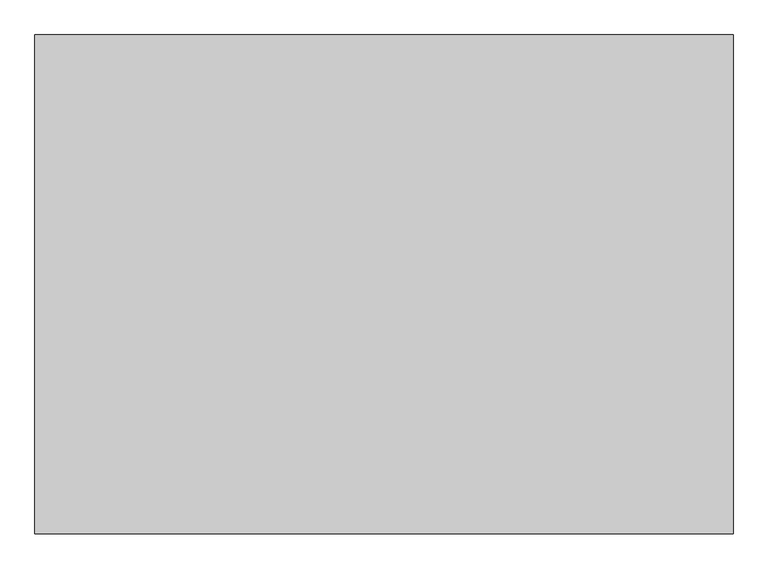
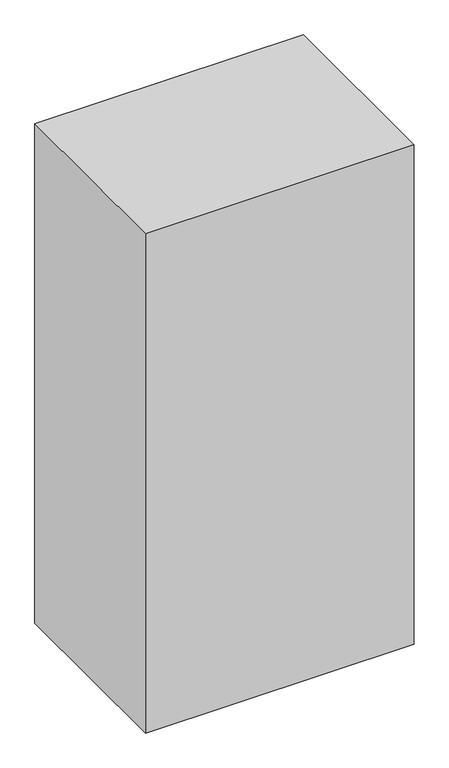
"""IFC4 building model written with IfcOpenShell, lengths in millimetres: proxy geometry, Space Planning Box_hec : Space Planning Box_hec."""

import ifcopenshell
import ifcopenshell.guid

model = None  # the IFC model being written
_history = None  # IfcOwnerHistory: only IFC2X3 demands one
_inside = {}  # id of a spatial element -> (the spatial element, [elements in it])
_under = {}  # id of a project, library or spatial element -> (it, [spatial elements below it])
_declared = {}  # id of a project -> (the project, [libraries it declares])
_typed = {}  # id of a type object -> (the type object, [elements of that type])
_made_of = {}  # id of a material, layer set ... -> (it, [elements and type objects made of it])


def new_model(schema):
    """Start an empty IFC model of exactly this schema.

    Asked for "IFC4X3", IfcOpenShell would pick the latest addendum, in which some entities
    have other attributes; the version numbers below select the first issue.
    IFC2X3 requires an IfcOwnerHistory on every rooted entity: one is made here for all.
    """
    global model, _history
    if schema == "IFC4X3":
        model = ifcopenshell.file(schema_version=(4, 3, 0, 0))
    else:
        model = ifcopenshell.file(schema=schema)
    _inside.clear()
    _under.clear()
    _declared.clear()
    _typed.clear()
    _made_of.clear()
    _history = None
    if model.schema == "IFC2X3":
        org = make("IfcOrganization", Name="unknown")
        user = make(
            "IfcPersonAndOrganization",
            ThePerson=make("IfcPerson", FamilyName="unknown"),
            TheOrganization=org,
        )
        app = make(
            "IfcApplication",
            ApplicationDeveloper=org,
            Version="unknown",
            ApplicationFullName="unknown",
            ApplicationIdentifier="unknown",
        )
        _history = make(
            "IfcOwnerHistory",
            OwningUser=user,
            OwningApplication=app,
            ChangeAction="ADDED",
            CreationDate=0,
        )
    return model


def make(cls, **values):
    """One entity of the class cls with the attributes given. An attribute that is None is left unset."""
    return model.create_entity(
        cls, **{name: value for name, value in values.items() if value is not None}
    )


def rooted(cls, **values):
    """An entity with a GlobalId (a new one), such as an element, a storey or a relation."""
    return make(cls, GlobalId=ifcopenshell.guid.new(), OwnerHistory=_history, **values)


def si_unit(unit_type, name, prefix=None):
    """IfcSIUnit, for example si_unit("LENGTHUNIT", "METRE", prefix="MILLI")."""
    return make("IfcSIUnit", UnitType=unit_type, Prefix=prefix, Name=name)


def assignment(units):
    """IfcUnitAssignment: the units of a project."""
    return None if units is None else make("IfcUnitAssignment", Units=units)


def point(xyz):
    """IfcCartesianPoint."""
    return None if xyz is None else make("IfcCartesianPoint", Coordinates=xyz)


def direction(xyz):
    """IfcDirection."""
    return None if xyz is None else make("IfcDirection", DirectionRatios=xyz)


def frame(location, z_axis=None, x_axis=None):
    """IfcAxis2Placement3D, a coordinate frame: its origin and axes. An axis left out is left unset."""
    return make(
        "IfcAxis2Placement3D",
        Location=point(location),
        Axis=direction(z_axis),
        RefDirection=direction(x_axis),
    )


def origin():
    """The frame at (0, 0, 0) with its axes left unset."""
    return frame((0.0, 0.0, 0.0))


def origin_with_axes():
    """The frame at (0, 0, 0) with the z axis (0, 0, 1) and the x axis (1, 0, 0) written out."""
    return frame((0.0, 0.0, 0.0), z_axis=(0.0, 0.0, 1.0), x_axis=(1.0, 0.0, 0.0))


def place(relative_to, where):
    """IfcLocalPlacement: puts the frame where relative to a parent placement (None: the world)."""
    return make(
        "IfcLocalPlacement", PlacementRelTo=relative_to, RelativePlacement=where
    )


def context(
    kind, dimensions, precision=None, world=None, true_north=None, identifier=None
):
    """IfcGeometricRepresentationContext, for example the 3D "Model" context."""
    return make(
        "IfcGeometricRepresentationContext",
        ContextIdentifier=identifier,
        ContextType=kind,
        CoordinateSpaceDimension=dimensions,
        Precision=precision,
        WorldCoordinateSystem=world,
        TrueNorth=true_north,
    )


def project(units=None, contexts=None):
    """IfcProject with its units and contexts."""
    return rooted(
        "IfcProject",
        Name="project",
        RepresentationContexts=contexts,
        UnitsInContext=assignment(units),
    )


def spatial(cls, under=None, at=None, **own):
    """A site, building, storey or space (cls), placed at a placement, below another one or the project."""
    s = rooted(cls, ObjectPlacement=at, **own)
    if under is not None:
        _under.setdefault(under.id(), (under, []))[1].append(s)
    return s


def polyline(points):
    """IfcPolyline through the points."""
    return make("IfcPolyline", Points=[point(p) for p in points])


def outline(outer, holes=None, kind="AREA"):
    """IfcArbitraryClosedProfileDef: a profile drawn as a closed curve; with holes, ...WithVoids."""
    if holes is None:
        return make("IfcArbitraryClosedProfileDef", ProfileType=kind, OuterCurve=outer)
    return make(
        "IfcArbitraryProfileDefWithVoids",
        ProfileType=kind,
        OuterCurve=outer,
        InnerCurves=holes,
    )


def extrude(swept, where, along, depth):
    """IfcExtrudedAreaSolid: the profile swept, set in the frame where, extruded along a direction by depth."""
    return make(
        "IfcExtrudedAreaSolid",
        SweptArea=swept,
        Position=where,
        ExtrudedDirection=direction(along),
        Depth=depth,
    )


def shape(context_of_items, identifier, shape_type, items):
    """IfcShapeRepresentation: the items that make up one representation, for example the "Body"."""
    return make(
        "IfcShapeRepresentation",
        ContextOfItems=context_of_items,
        RepresentationIdentifier=identifier,
        RepresentationType=shape_type,
        Items=items,
    )


def source(mapping_origin, context_of_items, identifier, shape_type, items):
    """IfcRepresentationMap: a shape defined once, which mapped items show again and again."""
    return make(
        "IfcRepresentationMap",
        MappingOrigin=mapping_origin,
        MappedRepresentation=shape(context_of_items, identifier, shape_type, items),
    )


def transform(
    local_origin,
    x_axis=None,
    y_axis=None,
    z_axis=None,
    scale=None,
    scale2=None,
    scale3=None,
    uniform=True,
):
    """IfcCartesianTransformationOperator3D, or its non-uniform kind. x_axis, y_axis, z_axis: its Axis1, 2, 3."""
    if uniform:
        return make(
            "IfcCartesianTransformationOperator3D",
            Axis1=direction(x_axis),
            Axis2=direction(y_axis),
            LocalOrigin=point(local_origin),
            Scale=scale,
            Axis3=direction(z_axis),
        )
    return make(
        "IfcCartesianTransformationOperator3DnonUniform",
        Axis1=direction(x_axis),
        Axis2=direction(y_axis),
        LocalOrigin=point(local_origin),
        Scale=scale,
        Axis3=direction(z_axis),
        Scale2=scale2,
        Scale3=scale3,
    )


def mapped(mapping_source, mapping_target):
    """IfcMappedItem: shows the shape of a source again, moved by a transform."""
    return make(
        "IfcMappedItem", MappingSource=mapping_source, MappingTarget=mapping_target
    )


def made_of(thing, what):
    """Note that an element or type object is made of a material, layer set ...; save() writes the relation."""
    if what is not None:
        _made_of.setdefault(what.id(), (what, []))[1].append(thing)
    return thing


def element(
    cls,
    number,
    at=None,
    inside=None,
    cuts=None,
    type_object=None,
    material=None,
    context=None,
    identifier="Body",
    shape_type=None,
    held_by="IfcProductDefinitionShape",
    body=None,
    shapes=None,
    **own,
):
    """One element of the class cls, such as IfcWall. Its Tag is "e" and its number.

    at: its placement. inside: the storey or other place that contains it. cuts: it is an
    opening in that element (IfcRelVoidsElement). A single representation is given by context,
    identifier, shape_type and body (its items); several are given by shapes. held_by: the class
    of the entity that holds the representations. save() writes the other relations.
    """
    e = rooted(cls, Tag="e%d" % number, ObjectPlacement=at, **own)
    if body is not None:
        shapes = [shape(context, identifier, shape_type, body)]
    if shapes is not None:
        e.Representation = make(held_by, Representations=shapes)
    if inside is not None:
        _inside.setdefault(inside.id(), (inside, []))[1].append(e)
    if cuts is not None:
        rooted(
            "IfcRelVoidsElement", RelatingBuildingElement=cuts, RelatedOpeningElement=e
        )
    if type_object is not None:
        _typed.setdefault(type_object.id(), (type_object, []))[1].append(e)
    return made_of(e, material)


def aggregate(whole, parts):
    """IfcRelAggregates: a whole, such as a stair, and the parts it consists of."""
    return rooted("IfcRelAggregates", RelatingObject=whole, RelatedObjects=parts)


def save(model, path):
    """Write the relations noted so far, then the file.

    IfcRelAggregates (storeys below a building ...), IfcRelContainedInSpatialStructure (elements
    in a storey), IfcRelDefinesByType, IfcRelAssociatesMaterial and IfcRelDeclares: one each for
    every whole, place, type object, material and project.
    """
    for whole, parts in _under.values():
        aggregate(whole, parts)
    for where, things in _inside.values():
        rooted(
            "IfcRelContainedInSpatialStructure",
            RelatedElements=things,
            RelatingStructure=where,
        )
    for kind, things in _typed.values():
        rooted("IfcRelDefinesByType", RelatedObjects=things, RelatingType=kind)
    for what, things in _made_of.values():
        rooted("IfcRelAssociatesMaterial", RelatedObjects=things, RelatingMaterial=what)
    for by, libraries in _declared.values():
        rooted("IfcRelDeclares", RelatingContext=by, RelatedDefinitions=libraries)
    model.write(path)


def generic_models_ee32b0c6(model_context):
    return source(origin(), model_context, "Body", "SweptSolid", [
        extrude(outline(polyline([(1400.0, 1000.0), (1400.0, -1000.0), (-1400.0, -1000.0), (-1400.0, 1000.0), (1400.0, 1000.0)])), origin_with_axes(), (0.0, 0.0, 1.0), 5500.0),
    ])


if __name__ == "__main__":
    model = new_model("IFC4")
    model_context = context("Model", 3, world=origin())
    ifc_project = project(units=[si_unit("LENGTHUNIT", "METRE", prefix="MILLI")], contexts=[model_context])
    site = spatial("IfcSite", under=ifc_project)
    building = spatial("IfcBuilding", under=site)
    placement = place(None, origin())
    generic_models_shape = generic_models_ee32b0c6(model_context)
    element("IfcBuildingElementProxy", 1, Name="Space Planning Box_hec : Space Planning Box_hec", ObjectType="Space Planning Box_hec : Space Planning Box_hec", at=placement, inside=building, context=model_context, shape_type="MappedRepresentation", body=[
        mapped(generic_models_shape, transform((0.0, 0.0, 0.0), x_axis=(1.0, 0.0, 0.0), y_axis=(0.0, 1.0, 0.0), z_axis=(0.0, 0.0, 1.0))),
    ])
    save(model, "model.ifc")

# Revit data of these elements
# Type "Space Planning Box_hec : Space Planning Box_hec"
#   Type Comments = "..."
#   Room Name [instance default] = "?"
#   Interior Finish [instance default] = ""
#   Exterior Finish [instance default] = ""
#   Department [instance default] = ""
#   Assembly Code = "..."
#   ceiling height [instance default] = 0
#   Width [instance default] = 1524 mm
#   Program Area [instance default] = 0.00 m²
#   Length [instance default] = 1524 mm
#   Height [instance default] = 1524 mm
#   Area [instance default] = 2.32258 m²
#   Fill Color [instance default] = Cyan
#   Default Elevation = 0
# Element 1 (IfcBuildingElementProxy, "Space Planning Box_hec : Space Planning Box_hec")
#   Room Name = "Shower"
#   Exterior Finish = "N/A..N/A,,EW2..N/A..N/A"
#   Department = "AR"
#   Width = 2800 mm
#   Program Area = 5.60 m²
#   Length = 2000 mm
#   Height = 5500 mm
#   Area = 5.60 m²
#   Materials on its faces: "Cyan"
# Materials
#   "Cyan": class "Generic", colour RGB 0 255 255, transparency 0.2, Cost = 0
